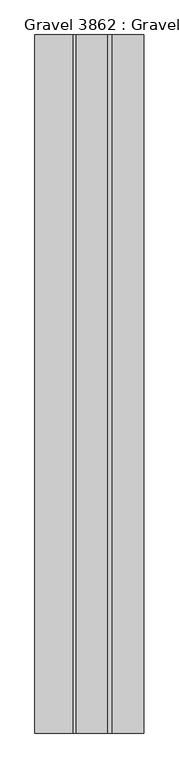
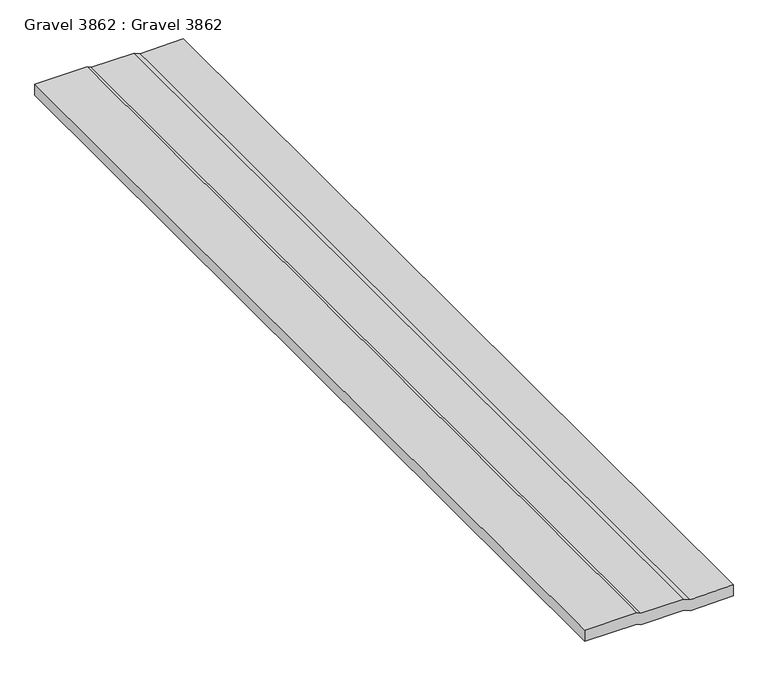
"""IFC4 building model written with IfcOpenShell, lengths in millimetres: proxy geometry, Gravel 3862 : Gravel 3862."""

import ifcopenshell
import ifcopenshell.guid

model = None  # the IFC model being written
_history = None  # IfcOwnerHistory: only IFC2X3 demands one
_inside = {}  # id of a spatial element -> (the spatial element, [elements in it])
_under = {}  # id of a project, library or spatial element -> (it, [spatial elements below it])
_declared = {}  # id of a project -> (the project, [libraries it declares])
_typed = {}  # id of a type object -> (the type object, [elements of that type])
_made_of = {}  # id of a material, layer set ... -> (it, [elements and type objects made of it])


def new_model(schema):
    """Start an empty IFC model of exactly this schema.

    Asked for "IFC4X3", IfcOpenShell would pick the latest addendum, in which some entities
    have other attributes; the version numbers below select the first issue.
    IFC2X3 requires an IfcOwnerHistory on every rooted entity: one is made here for all.
    """
    global model, _history
    if schema == "IFC4X3":
        model = ifcopenshell.file(schema_version=(4, 3, 0, 0))
    else:
        model = ifcopenshell.file(schema=schema)
    _inside.clear()
    _under.clear()
    _declared.clear()
    _typed.clear()
    _made_of.clear()
    _history = None
    if model.schema == "IFC2X3":
        org = make("IfcOrganization", Name="unknown")
        user = make(
            "IfcPersonAndOrganization",
            ThePerson=make("IfcPerson", FamilyName="unknown"),
            TheOrganization=org,
        )
        app = make(
            "IfcApplication",
            ApplicationDeveloper=org,
            Version="unknown",
            ApplicationFullName="unknown",
            ApplicationIdentifier="unknown",
        )
        _history = make(
            "IfcOwnerHistory",
            OwningUser=user,
            OwningApplication=app,
            ChangeAction="ADDED",
            CreationDate=0,
        )
    return model


def make(cls, **values):
    """One entity of the class cls with the attributes given. An attribute that is None is left unset."""
    return model.create_entity(
        cls, **{name: value for name, value in values.items() if value is not None}
    )


def rooted(cls, **values):
    """An entity with a GlobalId (a new one), such as an element, a storey or a relation."""
    return make(cls, GlobalId=ifcopenshell.guid.new(), OwnerHistory=_history, **values)


def si_unit(unit_type, name, prefix=None):
    """IfcSIUnit, for example si_unit("LENGTHUNIT", "METRE", prefix="MILLI")."""
    return make("IfcSIUnit", UnitType=unit_type, Prefix=prefix, Name=name)


def assignment(units):
    """IfcUnitAssignment: the units of a project."""
    return None if units is None else make("IfcUnitAssignment", Units=units)


def point(xyz):
    """IfcCartesianPoint."""
    return None if xyz is None else make("IfcCartesianPoint", Coordinates=xyz)


def direction(xyz):
    """IfcDirection."""
    return None if xyz is None else make("IfcDirection", DirectionRatios=xyz)


def frame(location, z_axis=None, x_axis=None):
    """IfcAxis2Placement3D, a coordinate frame: its origin and axes. An axis left out is left unset."""
    return make(
        "IfcAxis2Placement3D",
        Location=point(location),
        Axis=direction(z_axis),
        RefDirection=direction(x_axis),
    )


def origin():
    """The frame at (0, 0, 0) with its axes left unset."""
    return frame((0.0, 0.0, 0.0))


def place(relative_to, where):
    """IfcLocalPlacement: puts the frame where relative to a parent placement (None: the world)."""
    return make(
        "IfcLocalPlacement", PlacementRelTo=relative_to, RelativePlacement=where
    )


def context(
    kind, dimensions, precision=None, world=None, true_north=None, identifier=None
):
    """IfcGeometricRepresentationContext, for example the 3D "Model" context."""
    return make(
        "IfcGeometricRepresentationContext",
        ContextIdentifier=identifier,
        ContextType=kind,
        CoordinateSpaceDimension=dimensions,
        Precision=precision,
        WorldCoordinateSystem=world,
        TrueNorth=true_north,
    )


def project(units=None, contexts=None):
    """IfcProject with its units and contexts."""
    return rooted(
        "IfcProject",
        Name="project",
        RepresentationContexts=contexts,
        UnitsInContext=assignment(units),
    )


def spatial(cls, under=None, at=None, **own):
    """A site, building, storey or space (cls), placed at a placement, below another one or the project."""
    s = rooted(cls, ObjectPlacement=at, **own)
    if under is not None:
        _under.setdefault(under.id(), (under, []))[1].append(s)
    return s


def polyline(points):
    """IfcPolyline through the points."""
    return make("IfcPolyline", Points=[point(p) for p in points])


def outline(outer, holes=None, kind="AREA"):
    """IfcArbitraryClosedProfileDef: a profile drawn as a closed curve; with holes, ...WithVoids."""
    if holes is None:
        return make("IfcArbitraryClosedProfileDef", ProfileType=kind, OuterCurve=outer)
    return make(
        "IfcArbitraryProfileDefWithVoids",
        ProfileType=kind,
        OuterCurve=outer,
        InnerCurves=holes,
    )


def extrude(swept, where, along, depth):
    """IfcExtrudedAreaSolid: the profile swept, set in the frame where, extruded along a direction by depth."""
    return make(
        "IfcExtrudedAreaSolid",
        SweptArea=swept,
        Position=where,
        ExtrudedDirection=direction(along),
        Depth=depth,
    )


def shape(context_of_items, identifier, shape_type, items):
    """IfcShapeRepresentation: the items that make up one representation, for example the "Body"."""
    return make(
        "IfcShapeRepresentation",
        ContextOfItems=context_of_items,
        RepresentationIdentifier=identifier,
        RepresentationType=shape_type,
        Items=items,
    )


def source(mapping_origin, context_of_items, identifier, shape_type, items):
    """IfcRepresentationMap: a shape defined once, which mapped items show again and again."""
    return make(
        "IfcRepresentationMap",
        MappingOrigin=mapping_origin,
        MappedRepresentation=shape(context_of_items, identifier, shape_type, items),
    )


def transform(
    local_origin,
    x_axis=None,
    y_axis=None,
    z_axis=None,
    scale=None,
    scale2=None,
    scale3=None,
    uniform=True,
):
    """IfcCartesianTransformationOperator3D, or its non-uniform kind. x_axis, y_axis, z_axis: its Axis1, 2, 3."""
    if uniform:
        return make(
            "IfcCartesianTransformationOperator3D",
            Axis1=direction(x_axis),
            Axis2=direction(y_axis),
            LocalOrigin=point(local_origin),
            Scale=scale,
            Axis3=direction(z_axis),
        )
    return make(
        "IfcCartesianTransformationOperator3DnonUniform",
        Axis1=direction(x_axis),
        Axis2=direction(y_axis),
        LocalOrigin=point(local_origin),
        Scale=scale,
        Axis3=direction(z_axis),
        Scale2=scale2,
        Scale3=scale3,
    )


def mapped(mapping_source, mapping_target):
    """IfcMappedItem: shows the shape of a source again, moved by a transform."""
    return make(
        "IfcMappedItem", MappingSource=mapping_source, MappingTarget=mapping_target
    )


def made_of(thing, what):
    """Note that an element or type object is made of a material, layer set ...; save() writes the relation."""
    if what is not None:
        _made_of.setdefault(what.id(), (what, []))[1].append(thing)
    return thing


def element(
    cls,
    number,
    at=None,
    inside=None,
    cuts=None,
    type_object=None,
    material=None,
    context=None,
    identifier="Body",
    shape_type=None,
    held_by="IfcProductDefinitionShape",
    body=None,
    shapes=None,
    **own,
):
    """One element of the class cls, such as IfcWall. Its Tag is "e" and its number.

    at: its placement. inside: the storey or other place that contains it. cuts: it is an
    opening in that element (IfcRelVoidsElement). A single representation is given by context,
    identifier, shape_type and body (its items); several are given by shapes. held_by: the class
    of the entity that holds the representations. save() writes the other relations.
    """
    e = rooted(cls, Tag="e%d" % number, ObjectPlacement=at, **own)
    if body is not None:
        shapes = [shape(context, identifier, shape_type, body)]
    if shapes is not None:
        e.Representation = make(held_by, Representations=shapes)
    if inside is not None:
        _inside.setdefault(inside.id(), (inside, []))[1].append(e)
    if cuts is not None:
        rooted(
            "IfcRelVoidsElement", RelatingBuildingElement=cuts, RelatedOpeningElement=e
        )
    if type_object is not None:
        _typed.setdefault(type_object.id(), (type_object, []))[1].append(e)
    return made_of(e, material)


def aggregate(whole, parts):
    """IfcRelAggregates: a whole, such as a stair, and the parts it consists of."""
    return rooted("IfcRelAggregates", RelatingObject=whole, RelatedObjects=parts)


def save(model, path):
    """Write the relations noted so far, then the file.

    IfcRelAggregates (storeys below a building ...), IfcRelContainedInSpatialStructure (elements
    in a storey), IfcRelDefinesByType, IfcRelAssociatesMaterial and IfcRelDeclares: one each for
    every whole, place, type object, material and project.
    """
    for whole, parts in _under.values():
        aggregate(whole, parts)
    for where, things in _inside.values():
        rooted(
            "IfcRelContainedInSpatialStructure",
            RelatedElements=things,
            RelatingStructure=where,
        )
    for kind, things in _typed.values():
        rooted("IfcRelDefinesByType", RelatedObjects=things, RelatingType=kind)
    for what, things in _made_of.values():
        rooted("IfcRelAssociatesMaterial", RelatedObjects=things, RelatingMaterial=what)
    for by, libraries in _declared.values():
        rooted("IfcRelDeclares", RelatingContext=by, RelatedDefinitions=libraries)
    model.write(path)


def gravel_3862_gravel_3862_052f081c(model_context):
    return source(origin(), model_context, "Body", "SweptSolid", [
        extrude(outline(polyline([(40274.2359464, -4902.3767758), (40269.9546964, -4893.6663265), (40269.9546964, -4803.0794125), (40264.2272344, -4790.2347731), (40265.8726651, -4699.8063764), (40290.6109464, -4699.8063764), (40288.9655157, -4790.2347731), (40294.6929777, -4803.0794125), (40294.6929777, -4893.6663265), (40298.9742277, -4902.3767758), (40298.9742277, -5011.8762875), (40274.2359464, -5011.8762875), (40274.2359464, -4902.3767758)])), frame((0.0, -1052.6406573, 0.0), z_axis=(0.0, 1.0, 0.0), x_axis=(0.0, 0.0, 1.0)), (0.0, 0.0, 1.0), 2000.0),
    ])


if __name__ == "__main__":
    model = new_model("IFC4")
    model_context = context("Model", 3, world=origin())
    ifc_project = project(units=[si_unit("LENGTHUNIT", "METRE", prefix="MILLI")], contexts=[model_context])
    site = spatial("IfcSite", under=ifc_project)
    building = spatial("IfcBuilding", under=site)
    placement = place(None, origin())
    gravel_3862_gravel_3862_shape = gravel_3862_gravel_3862_052f081c(model_context)
    element("IfcBuildingElementProxy", 1, Name="Gravel 3862 : Gravel 3862", ObjectType="Gravel 3862 : Gravel 3862", at=placement, inside=building, context=model_context, shape_type="MappedRepresentation", body=[
        mapped(gravel_3862_gravel_3862_shape, transform((0.0, 0.0, 0.0), x_axis=(1.0, 0.0, 0.0), y_axis=(0.0, 1.0, 0.0), z_axis=(0.0, 0.0, 1.0))),
    ])
    save(model, "model.ifc")

# Revit data of these elements
# Type "Gravel 3862 : Gravel 3862"
#   NameOverride = "Gravel"
# Element 1 (IfcBuildingElementProxy, "Gravel 3862 : Gravel 3862")
#   Materials on its faces: "GRAVEL BALLAST"
# Materials
#   "GRAVEL BALLAST": class "Unassigned", colour RGB 128 128 128, transparency 0, Cost = 0
